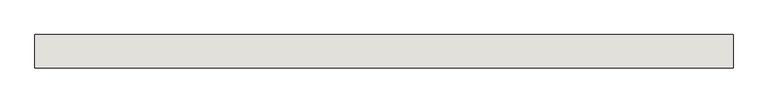
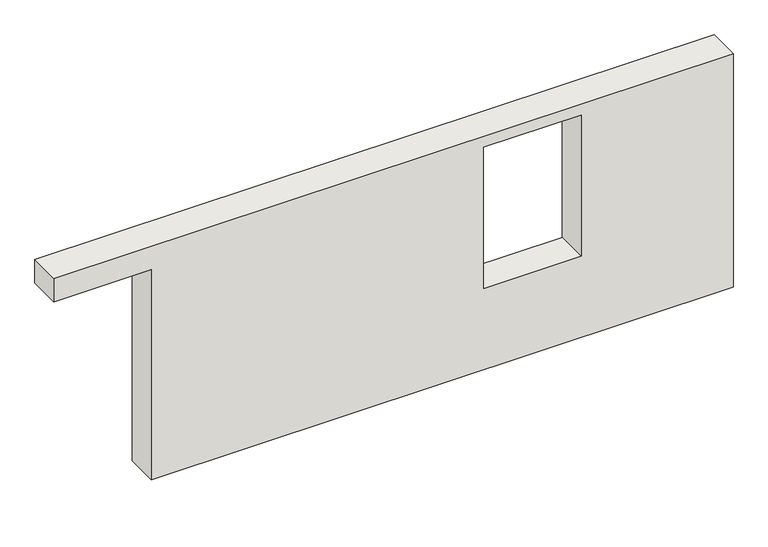
"""IFC4 building model written with IfcOpenShell, lengths in millimetres: wall geometry, 0_3d."""

import ifcopenshell
import ifcopenshell.guid

model = None  # the IFC model being written
_history = None  # IfcOwnerHistory: only IFC2X3 demands one
_inside = {}  # id of a spatial element -> (the spatial element, [elements in it])
_under = {}  # id of a project, library or spatial element -> (it, [spatial elements below it])
_declared = {}  # id of a project -> (the project, [libraries it declares])
_typed = {}  # id of a type object -> (the type object, [elements of that type])
_made_of = {}  # id of a material, layer set ... -> (it, [elements and type objects made of it])


def new_model(schema):
    """Start an empty IFC model of exactly this schema.

    Asked for "IFC4X3", IfcOpenShell would pick the latest addendum, in which some entities
    have other attributes; the version numbers below select the first issue.
    IFC2X3 requires an IfcOwnerHistory on every rooted entity: one is made here for all.
    """
    global model, _history
    if schema == "IFC4X3":
        model = ifcopenshell.file(schema_version=(4, 3, 0, 0))
    else:
        model = ifcopenshell.file(schema=schema)
    _inside.clear()
    _under.clear()
    _declared.clear()
    _typed.clear()
    _made_of.clear()
    _history = None
    if model.schema == "IFC2X3":
        org = make("IfcOrganization", Name="unknown")
        user = make(
            "IfcPersonAndOrganization",
            ThePerson=make("IfcPerson", FamilyName="unknown"),
            TheOrganization=org,
        )
        app = make(
            "IfcApplication",
            ApplicationDeveloper=org,
            Version="unknown",
            ApplicationFullName="unknown",
            ApplicationIdentifier="unknown",
        )
        _history = make(
            "IfcOwnerHistory",
            OwningUser=user,
            OwningApplication=app,
            ChangeAction="ADDED",
            CreationDate=0,
        )
    return model


def make(cls, **values):
    """One entity of the class cls with the attributes given. An attribute that is None is left unset."""
    return model.create_entity(
        cls, **{name: value for name, value in values.items() if value is not None}
    )


def rooted(cls, **values):
    """An entity with a GlobalId (a new one), such as an element, a storey or a relation."""
    return make(cls, GlobalId=ifcopenshell.guid.new(), OwnerHistory=_history, **values)


def si_unit(unit_type, name, prefix=None):
    """IfcSIUnit, for example si_unit("LENGTHUNIT", "METRE", prefix="MILLI")."""
    return make("IfcSIUnit", UnitType=unit_type, Prefix=prefix, Name=name)


def assignment(units):
    """IfcUnitAssignment: the units of a project."""
    return None if units is None else make("IfcUnitAssignment", Units=units)


def point(xyz):
    """IfcCartesianPoint."""
    return None if xyz is None else make("IfcCartesianPoint", Coordinates=xyz)


def direction(xyz):
    """IfcDirection."""
    return None if xyz is None else make("IfcDirection", DirectionRatios=xyz)


def frame(location, z_axis=None, x_axis=None):
    """IfcAxis2Placement3D, a coordinate frame: its origin and axes. An axis left out is left unset."""
    return make(
        "IfcAxis2Placement3D",
        Location=point(location),
        Axis=direction(z_axis),
        RefDirection=direction(x_axis),
    )


def origin():
    """The frame at (0, 0, 0) with its axes left unset."""
    return frame((0.0, 0.0, 0.0))


def place(relative_to, where):
    """IfcLocalPlacement: puts the frame where relative to a parent placement (None: the world)."""
    return make(
        "IfcLocalPlacement", PlacementRelTo=relative_to, RelativePlacement=where
    )


def context(
    kind, dimensions, precision=None, world=None, true_north=None, identifier=None
):
    """IfcGeometricRepresentationContext, for example the 3D "Model" context."""
    return make(
        "IfcGeometricRepresentationContext",
        ContextIdentifier=identifier,
        ContextType=kind,
        CoordinateSpaceDimension=dimensions,
        Precision=precision,
        WorldCoordinateSystem=world,
        TrueNorth=true_north,
    )


def project(units=None, contexts=None):
    """IfcProject with its units and contexts."""
    return rooted(
        "IfcProject",
        Name="project",
        RepresentationContexts=contexts,
        UnitsInContext=assignment(units),
    )


def spatial(cls, under=None, at=None, **own):
    """A site, building, storey or space (cls), placed at a placement, below another one or the project."""
    s = rooted(cls, ObjectPlacement=at, **own)
    if under is not None:
        _under.setdefault(under.id(), (under, []))[1].append(s)
    return s


def polyline(points):
    """IfcPolyline through the points."""
    return make("IfcPolyline", Points=[point(p) for p in points])


def outline(outer, holes=None, kind="AREA"):
    """IfcArbitraryClosedProfileDef: a profile drawn as a closed curve; with holes, ...WithVoids."""
    if holes is None:
        return make("IfcArbitraryClosedProfileDef", ProfileType=kind, OuterCurve=outer)
    return make(
        "IfcArbitraryProfileDefWithVoids",
        ProfileType=kind,
        OuterCurve=outer,
        InnerCurves=holes,
    )


def extrude(swept, where, along, depth):
    """IfcExtrudedAreaSolid: the profile swept, set in the frame where, extruded along a direction by depth."""
    return make(
        "IfcExtrudedAreaSolid",
        SweptArea=swept,
        Position=where,
        ExtrudedDirection=direction(along),
        Depth=depth,
    )


def shape(context_of_items, identifier, shape_type, items):
    """IfcShapeRepresentation: the items that make up one representation, for example the "Body"."""
    return make(
        "IfcShapeRepresentation",
        ContextOfItems=context_of_items,
        RepresentationIdentifier=identifier,
        RepresentationType=shape_type,
        Items=items,
    )


def source(mapping_origin, context_of_items, identifier, shape_type, items):
    """IfcRepresentationMap: a shape defined once, which mapped items show again and again."""
    return make(
        "IfcRepresentationMap",
        MappingOrigin=mapping_origin,
        MappedRepresentation=shape(context_of_items, identifier, shape_type, items),
    )


def transform(
    local_origin,
    x_axis=None,
    y_axis=None,
    z_axis=None,
    scale=None,
    scale2=None,
    scale3=None,
    uniform=True,
):
    """IfcCartesianTransformationOperator3D, or its non-uniform kind. x_axis, y_axis, z_axis: its Axis1, 2, 3."""
    if uniform:
        return make(
            "IfcCartesianTransformationOperator3D",
            Axis1=direction(x_axis),
            Axis2=direction(y_axis),
            LocalOrigin=point(local_origin),
            Scale=scale,
            Axis3=direction(z_axis),
        )
    return make(
        "IfcCartesianTransformationOperator3DnonUniform",
        Axis1=direction(x_axis),
        Axis2=direction(y_axis),
        LocalOrigin=point(local_origin),
        Scale=scale,
        Axis3=direction(z_axis),
        Scale2=scale2,
        Scale3=scale3,
    )


def mapped(mapping_source, mapping_target):
    """IfcMappedItem: shows the shape of a source again, moved by a transform."""
    return make(
        "IfcMappedItem", MappingSource=mapping_source, MappingTarget=mapping_target
    )


def made_of(thing, what):
    """Note that an element or type object is made of a material, layer set ...; save() writes the relation."""
    if what is not None:
        _made_of.setdefault(what.id(), (what, []))[1].append(thing)
    return thing


def element(
    cls,
    number,
    at=None,
    inside=None,
    cuts=None,
    type_object=None,
    material=None,
    context=None,
    identifier="Body",
    shape_type=None,
    held_by="IfcProductDefinitionShape",
    body=None,
    shapes=None,
    **own,
):
    """One element of the class cls, such as IfcWall. Its Tag is "e" and its number.

    at: its placement. inside: the storey or other place that contains it. cuts: it is an
    opening in that element (IfcRelVoidsElement). A single representation is given by context,
    identifier, shape_type and body (its items); several are given by shapes. held_by: the class
    of the entity that holds the representations. save() writes the other relations.
    """
    e = rooted(cls, Tag="e%d" % number, ObjectPlacement=at, **own)
    if body is not None:
        shapes = [shape(context, identifier, shape_type, body)]
    if shapes is not None:
        e.Representation = make(held_by, Representations=shapes)
    if inside is not None:
        _inside.setdefault(inside.id(), (inside, []))[1].append(e)
    if cuts is not None:
        rooted(
            "IfcRelVoidsElement", RelatingBuildingElement=cuts, RelatedOpeningElement=e
        )
    if type_object is not None:
        _typed.setdefault(type_object.id(), (type_object, []))[1].append(e)
    return made_of(e, material)


def aggregate(whole, parts):
    """IfcRelAggregates: a whole, such as a stair, and the parts it consists of."""
    return rooted("IfcRelAggregates", RelatingObject=whole, RelatedObjects=parts)


def save(model, path):
    """Write the relations noted so far, then the file.

    IfcRelAggregates (storeys below a building ...), IfcRelContainedInSpatialStructure (elements
    in a storey), IfcRelDefinesByType, IfcRelAssociatesMaterial and IfcRelDeclares: one each for
    every whole, place, type object, material and project.
    """
    for whole, parts in _under.values():
        aggregate(whole, parts)
    for where, things in _inside.values():
        rooted(
            "IfcRelContainedInSpatialStructure",
            RelatedElements=things,
            RelatingStructure=where,
        )
    for kind, things in _typed.values():
        rooted("IfcRelDefinesByType", RelatedObjects=things, RelatingType=kind)
    for what, things in _made_of.values():
        rooted("IfcRelAssociatesMaterial", RelatedObjects=things, RelatingMaterial=what)
    for by, libraries in _declared.values():
        rooted("IfcRelDeclares", RelatingContext=by, RelatedDefinitions=libraries)
    model.write(path)


def wall_3b8d152a(model_context):
    return source(origin(), model_context, "Body", "SweptSolid", [
        extrude(outline(polyline([(2590.0, 0.0), (2590.0, 1135.0), (0.0, 1135.0), (0.0, 7920.0), (2880.0, 7920.0), (2880.0, 0.0), (2590.0, 0.0)]), holes=[polyline([(1000.0, 5015.0), (2740.0, 5015.0), (2740.0, 6150.0), (1000.0, 6150.0), (1000.0, 5015.0)])]), frame((0.0, 0.0, 0.0), z_axis=(0.0, 1.0, 0.0), x_axis=(0.0, 0.0, 1.0)), (0.0, 0.0, 1.0), 380.0),
    ])


if __name__ == "__main__":
    model = new_model("IFC4")
    model_context = context("Model", 3, world=origin())
    ifc_project = project(units=[si_unit("LENGTHUNIT", "METRE", prefix="MILLI")], contexts=[model_context])
    site = spatial("IfcSite", under=ifc_project)
    building = spatial("IfcBuilding", under=site)
    placement = place(None, origin())
    wall_shape = wall_3b8d152a(model_context)
    element("IfcWall", 1, ObjectType="0_3d", at=placement, inside=building, context=model_context, shape_type="MappedRepresentation", body=[
        mapped(wall_shape, transform((0.0, 0.0, 0.0), x_axis=(1.0, 0.0, 0.0), y_axis=(0.0, 1.0, 0.0), z_axis=(0.0, 0.0, 1.0))),
    ])
    save(model, "model.ifc")

# Revit data of these elements
# Element 1 (IfcWall, "0_3d")
#   Materials on its faces: "holzschalung"
# Materials
#   "holzschalung": class "Unassigned", colour RGB 128 128 128, transparency 0
